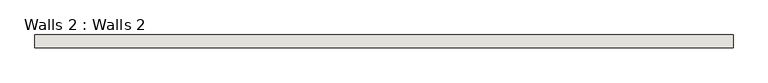
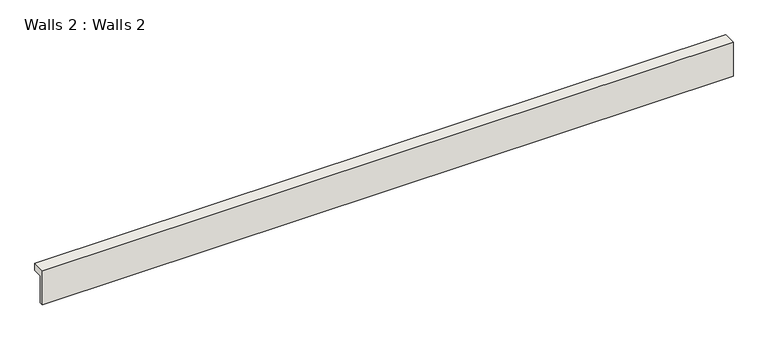
"""IFC4 building model written with IfcOpenShell, lengths in millimetres: wall geometry, Walls 2 : Walls 2."""

from ifc_helpers import new_model, si_unit, frame, origin, place, context, project, spatial, polyline, outline, extrude, source, transform, mapped, element, save


def walls_2_walls_2_429879ab(model_context):
    return source(origin(), model_context, "Body", "SweptSolid", [
        extrude(outline(polyline([(-1873.6830088, 6808.8866945), (-1746.6830088, 6808.8866945), (-1746.6830088, 6732.6866945), (-1840.8193734, 6732.6866945), (-1840.8193734, 6453.2866945), (-1873.6830088, 6453.2866945), (-1873.6830088, 6808.8866945)])), frame((25761.6402986, 0.0, 0.0), z_axis=(1.0, 0.0, 0.0), x_axis=(0.0, 1.0, 0.0)), (0.0, 0.0, 1.0), 6816.725),
    ])


if __name__ == "__main__":
    model = new_model("IFC4")
    model_context = context("Model", 3, world=origin())
    ifc_project = project(units=[si_unit("LENGTHUNIT", "METRE", prefix="MILLI")], contexts=[model_context])
    site = spatial("IfcSite", under=ifc_project)
    building = spatial("IfcBuilding", under=site)
    placement = place(None, origin())
    walls_2_walls_2_shape = walls_2_walls_2_429879ab(model_context)
    element("IfcWall", 1, ObjectType="Walls 2 : Walls 2", at=placement, inside=building, context=model_context, shape_type="MappedRepresentation", body=[
        mapped(walls_2_walls_2_shape, transform((0.0, 0.0, 0.0), x_axis=(1.0, 0.0, 0.0), y_axis=(0.0, 1.0, 0.0), z_axis=(0.0, 0.0, 1.0))),
    ])
    save(model, "model.ifc")

# Revit data of these elements
# Element 1 (IfcWall, "Walls 2 : Walls 2")
#   Materials on its faces: "Trim"
# Materials
#   "Trim": class "Wood", colour RGB 250 251 245, transparency 0, Cost = 0
